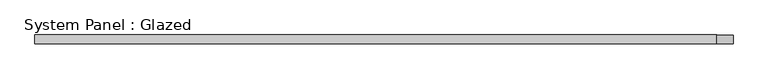
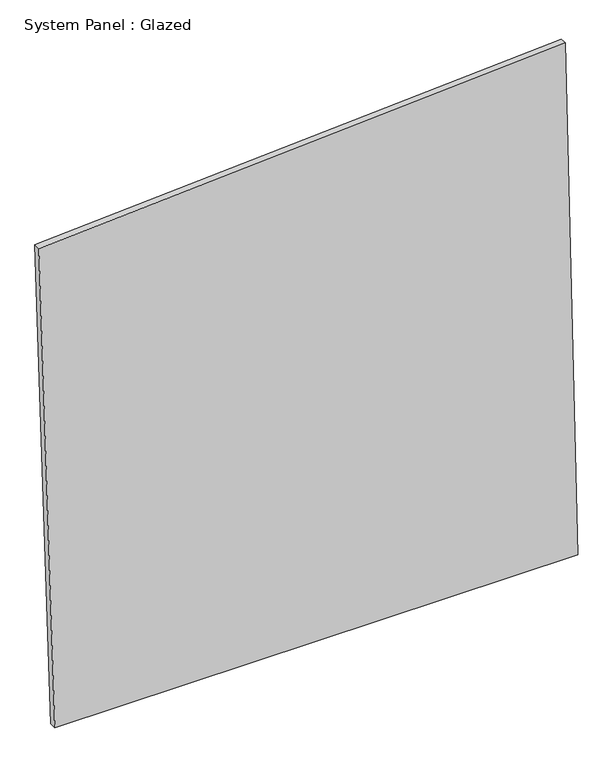
"""IFC4 building model written with IfcOpenShell, lengths in millimetres: plate geometry, System Panel : Glazed."""

from ifc_helpers import new_model, si_unit, frame, origin, place, context, project, spatial, polyline, outline, extrude, source, transform, mapped, element, save


def system_panel_glazed_31f0a782(model_context):
    return source(origin(), model_context, "Body", "SweptSolid", [
        extrude(outline(polyline([(0.0, -928.0385226), (0.0, 986.4208083), (1996.1252593, 940.8873527), (1874.9814945, -986.4208083), (0.0, -928.0385226)])), frame((0.0, -49.5, 0.0), z_axis=(0.0, 1.0, 0.0), x_axis=(0.0, 0.0, 1.0)), (0.0, 0.0, 1.0), 25.0),
    ])


if __name__ == "__main__":
    model = new_model("IFC4")
    model_context = context("Model", 3, world=origin())
    ifc_project = project(units=[si_unit("LENGTHUNIT", "METRE", prefix="MILLI")], contexts=[model_context])
    site = spatial("IfcSite", under=ifc_project)
    building = spatial("IfcBuilding", under=site)
    placement = place(None, origin())
    system_panel_glazed_shape = system_panel_glazed_31f0a782(model_context)
    element("IfcPlate", 1, ObjectType="System Panel : Glazed", at=placement, inside=building, context=model_context, shape_type="MappedRepresentation", body=[
        mapped(system_panel_glazed_shape, transform((0.0, 0.0, 0.0), x_axis=(1.0, 0.0, 0.0), y_axis=(0.0, 1.0, 0.0), z_axis=(0.0, 0.0, 1.0))),
    ])
    save(model, "model.ifc")

# Revit data of these elements
# Element 1 (IfcPlate, "System Panel : Glazed")
#   Materials on its faces: "Glass, Clear Glazing"
# Materials
#   "Glass, Clear Glazing": class "Glass", colour RGB 247 249 248, transparency 0.85, Description = "Clear glazing", Cost = 0
